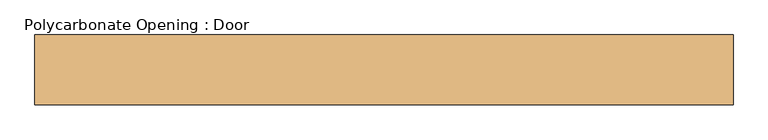
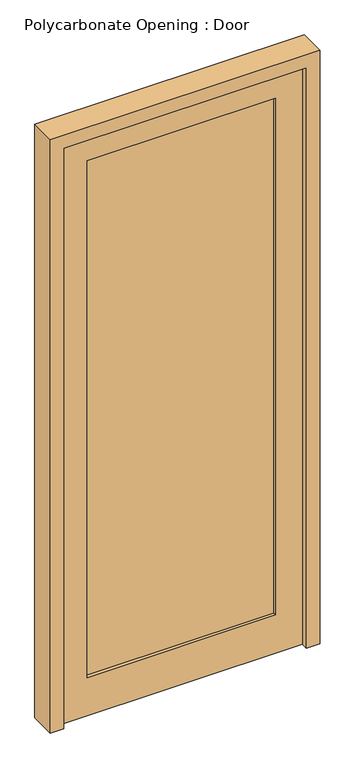
"""IFC4 building model written with IfcOpenShell, lengths in millimetres: door geometry, Polycarbonate Opening : Door."""

from ifc_helpers import new_model, si_unit, frame, origin, place, context, project, spatial, polyline, outline, extrude, source, transform, mapped, element, save


def polycarbonate_opening_door_7723b8a8(model_context):
    return source(origin(), model_context, "Body", "SweptSolid", [
        extrude(outline(polyline([(457.2, 0.0), (457.2, -25.4), (-457.2, -25.4), (-457.2, 0.0), (457.2, 0.0)])), frame((0.0, 0.0, 50.8), z_axis=(0.0, 0.0, 1.0), x_axis=(1.0, 0.0, 0.0)), (0.0, 0.0, 1.0), 2260.6),
        extrude(outline(polyline([(2311.4, -457.2), (0.0, -457.2), (0.0, 457.2), (2311.4, 457.2), (2311.4, -457.2)]), holes=[polyline([(152.4, 355.6), (152.4, -355.6), (2209.8, -355.6), (2209.8, 355.6), (152.4, 355.6)])]), frame((0.0, -38.1, 0.0), z_axis=(0.0, 1.0, 0.0), x_axis=(0.0, 0.0, 1.0)), (0.0, 0.0, 1.0), 50.8),
        extrude(outline(polyline([(2362.2, 508.0), (2362.2, -508.0), (0.0, -508.0), (0.0, -457.2), (2311.4, -457.2), (2311.4, 457.2), (0.0, 457.2), (0.0, 508.0), (2362.2, 508.0)])), frame((0.0, -63.5, 0.0), z_axis=(0.0, 1.0, 0.0), x_axis=(0.0, 0.0, 1.0)), (0.0, 0.0, 1.0), 101.6),
    ])


if __name__ == "__main__":
    model = new_model("IFC4")
    model_context = context("Model", 3, world=origin())
    ifc_project = project(units=[si_unit("LENGTHUNIT", "METRE", prefix="MILLI")], contexts=[model_context])
    site = spatial("IfcSite", under=ifc_project)
    building = spatial("IfcBuilding", under=site)
    placement = place(None, origin())
    polycarbonate_opening_door_shape = polycarbonate_opening_door_7723b8a8(model_context)
    element("IfcDoor", 1, ObjectType="Polycarbonate Opening : Door", at=placement, inside=building, context=model_context, shape_type="MappedRepresentation", body=[
        mapped(polycarbonate_opening_door_shape, transform((0.0, 0.0, 0.0), x_axis=(1.0, 0.0, 0.0), y_axis=(0.0, 1.0, 0.0), z_axis=(0.0, 0.0, 1.0))),
    ])
    save(model, "model.ifc")

# Revit data of these elements
# Type "Polycarbonate Opening : Door"
#   Type Mark = "60"
#   Analytic Construction = "<None>"
#   offset [instance default] = 0' - 0 1/2"
#   Stile = 0' - 4"
#   Mullion Width = 0' - 2"
#   Mullion Depth = 0' - 4"
#   Opening Size [instance default] = 5' - 1.50212"
#   Door Width [instance default] = 5' - 1.50212"
#   Window ON/OFF = yes
#   Door On/Off = no
#   Mullion Material = ALUMINUM STOREFRONT
#   Glass Material = INSULATED GLAZING
#   Door Material = ALUMINUM STOREFRONT
# Element 1 (IfcDoor, "Polycarbonate Opening : Door")
#   Materials on its faces: "ALUMINUM STOREFRONT", "INSULATED GLAZING"
# Materials
#   "ALUMINUM STOREFRONT": class "Metal", colour RGB 244 244 244, transparency 0, Description = "Aluminum 6061", Cost = 0
#   "INSULATED GLAZING": class "Glass", colour RGB 196 205 210, transparency 0.85, Description = "Soda Lime Glass", Cost = 0
